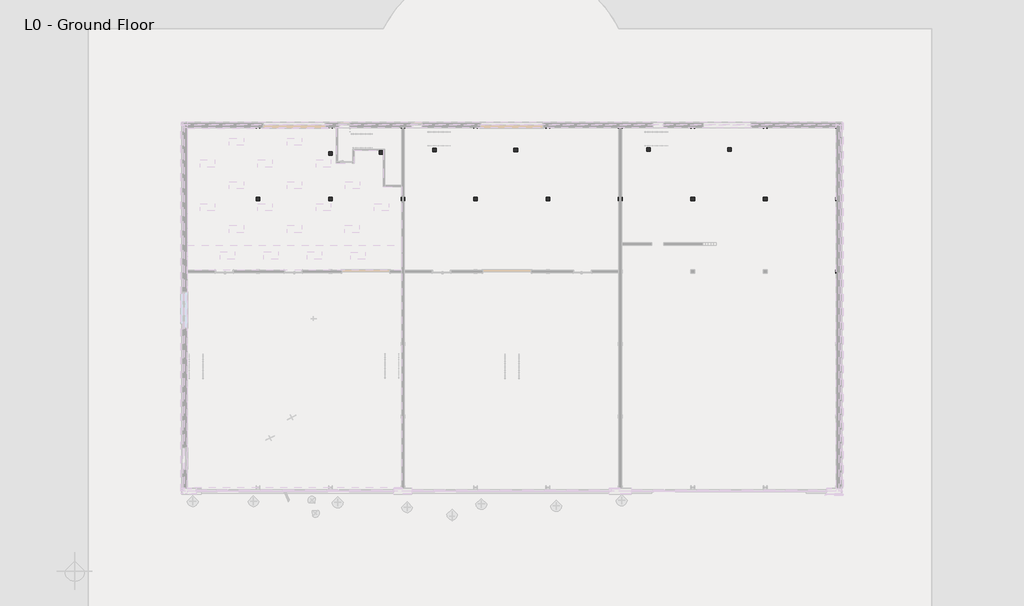
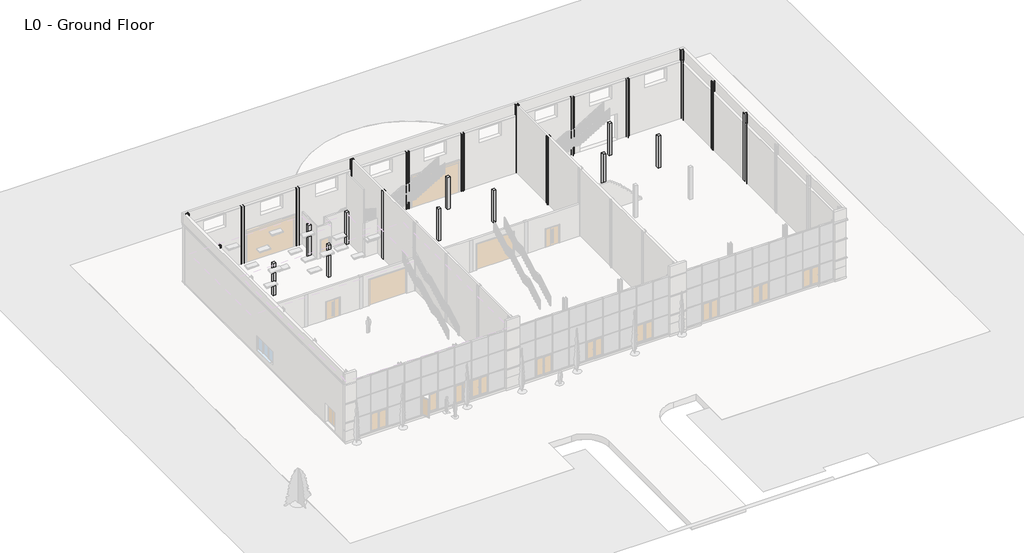
# One storey, part 7 of 14: 27 columns, 22 slabs, 2 footings.
"""IFC4 building model written with IfcOpenShell, lengths in millimetres."""

import ifcopenshell
import ifcopenshell.guid

model = None  # the IFC model being written
_history = None  # IfcOwnerHistory: only IFC2X3 demands one
_inside = {}  # id of a spatial element -> (the spatial element, [elements in it])
_under = {}  # id of a project, library or spatial element -> (it, [spatial elements below it])
_declared = {}  # id of a project -> (the project, [libraries it declares])
_typed = {}  # id of a type object -> (the type object, [elements of that type])
_made_of = {}  # id of a material, layer set ... -> (it, [elements and type objects made of it])


def new_model(schema):
    """Start an empty IFC model of exactly this schema.

    Asked for "IFC4X3", IfcOpenShell would pick the latest addendum, in which some entities
    have other attributes; the version numbers below select the first issue.
    IFC2X3 requires an IfcOwnerHistory on every rooted entity: one is made here for all.
    """
    global model, _history
    if schema == "IFC4X3":
        model = ifcopenshell.file(schema_version=(4, 3, 0, 0))
    else:
        model = ifcopenshell.file(schema=schema)
    _inside.clear()
    _under.clear()
    _declared.clear()
    _typed.clear()
    _made_of.clear()
    _history = None
    if model.schema == "IFC2X3":
        org = make("IfcOrganization", Name="unknown")
        user = make(
            "IfcPersonAndOrganization",
            ThePerson=make("IfcPerson", FamilyName="unknown"),
            TheOrganization=org,
        )
        app = make(
            "IfcApplication",
            ApplicationDeveloper=org,
            Version="unknown",
            ApplicationFullName="unknown",
            ApplicationIdentifier="unknown",
        )
        _history = make(
            "IfcOwnerHistory",
            OwningUser=user,
            OwningApplication=app,
            ChangeAction="ADDED",
            CreationDate=0,
        )
    return model


def make(cls, **values):
    """One entity of the class cls with the attributes given. An attribute that is None is left unset."""
    return model.create_entity(
        cls, **{name: value for name, value in values.items() if value is not None}
    )


def rooted(cls, **values):
    """An entity with a GlobalId (a new one), such as an element, a storey or a relation."""
    return make(cls, GlobalId=ifcopenshell.guid.new(), OwnerHistory=_history, **values)


def si_unit(unit_type, name, prefix=None):
    """IfcSIUnit, for example si_unit("LENGTHUNIT", "METRE", prefix="MILLI")."""
    return make("IfcSIUnit", UnitType=unit_type, Prefix=prefix, Name=name)


def assignment(units):
    """IfcUnitAssignment: the units of a project."""
    return None if units is None else make("IfcUnitAssignment", Units=units)


def point(xyz):
    """IfcCartesianPoint."""
    return None if xyz is None else make("IfcCartesianPoint", Coordinates=xyz)


def direction(xyz):
    """IfcDirection."""
    return None if xyz is None else make("IfcDirection", DirectionRatios=xyz)


def frame(location, z_axis=None, x_axis=None):
    """IfcAxis2Placement3D, a coordinate frame: its origin and axes. An axis left out is left unset."""
    return make(
        "IfcAxis2Placement3D",
        Location=point(location),
        Axis=direction(z_axis),
        RefDirection=direction(x_axis),
    )


def frame_2d(location, x_axis=None):
    """IfcAxis2Placement2D, a coordinate frame in the plane: its origin and x axis."""
    return make(
        "IfcAxis2Placement2D", Location=point(location), RefDirection=direction(x_axis)
    )


def origin():
    """The frame at (0, 0, 0) with its axes left unset."""
    return frame((0.0, 0.0, 0.0))


def place(relative_to, where):
    """IfcLocalPlacement: puts the frame where relative to a parent placement (None: the world)."""
    return make(
        "IfcLocalPlacement", PlacementRelTo=relative_to, RelativePlacement=where
    )


def context(
    kind, dimensions, precision=None, world=None, true_north=None, identifier=None
):
    """IfcGeometricRepresentationContext, for example the 3D "Model" context."""
    return make(
        "IfcGeometricRepresentationContext",
        ContextIdentifier=identifier,
        ContextType=kind,
        CoordinateSpaceDimension=dimensions,
        Precision=precision,
        WorldCoordinateSystem=world,
        TrueNorth=true_north,
    )


def project(units=None, contexts=None):
    """IfcProject with its units and contexts."""
    return rooted(
        "IfcProject",
        Name="project",
        RepresentationContexts=contexts,
        UnitsInContext=assignment(units),
    )


def spatial(cls, under=None, at=None, **own):
    """A site, building, storey or space (cls), placed at a placement, below another one or the project."""
    s = rooted(cls, ObjectPlacement=at, **own)
    if under is not None:
        _under.setdefault(under.id(), (under, []))[1].append(s)
    return s


def polyline(points):
    """IfcPolyline through the points."""
    return make("IfcPolyline", Points=[point(p) for p in points])


def circle_curve(where, radius):
    """IfcCircle in the frame where."""
    return make("IfcCircle", Position=where, Radius=radius)


def trimmed(basis, trim1, trim2, sense, master):
    """IfcTrimmedCurve: the piece of a basis curve between two trims."""
    return make(
        "IfcTrimmedCurve",
        BasisCurve=basis,
        Trim1=trim1,
        Trim2=trim2,
        SenseAgreement=sense,
        MasterRepresentation=master,
    )


def segment(curve, same_sense, transition):
    """IfcCompositeCurveSegment."""
    return make(
        "IfcCompositeCurveSegment",
        Transition=transition,
        SameSense=same_sense,
        ParentCurve=curve,
    )


def composite_curve(segments, self_intersect=None):
    """IfcCompositeCurve: segments joined end to end."""
    return make("IfcCompositeCurve", Segments=segments, SelfIntersect=self_intersect)


def outline(outer, holes=None, kind="AREA"):
    """IfcArbitraryClosedProfileDef: a profile drawn as a closed curve; with holes, ...WithVoids."""
    if holes is None:
        return make("IfcArbitraryClosedProfileDef", ProfileType=kind, OuterCurve=outer)
    return make(
        "IfcArbitraryProfileDefWithVoids",
        ProfileType=kind,
        OuterCurve=outer,
        InnerCurves=holes,
    )


def extrude(swept, where, along, depth):
    """IfcExtrudedAreaSolid: the profile swept, set in the frame where, extruded along a direction by depth."""
    return make(
        "IfcExtrudedAreaSolid",
        SweptArea=swept,
        Position=where,
        ExtrudedDirection=direction(along),
        Depth=depth,
    )


def faces_of(points, faces, orient=None, outer=None):
    """IfcFace entities. A face is a list of loops; a loop is a list of indices into points, from 0.

    orient and outer hold one flag for each loop. By default every Orientation is true, the
    first loop of a face is its IfcFaceOuterBound and the others are IfcFaceBound.
    """
    made = []
    for i, loops in enumerate(faces):
        bounds = []
        for j, loop in enumerate(loops):
            is_outer = j == 0 if outer is None else outer[i][j]
            bounds.append(
                make(
                    "IfcFaceOuterBound" if is_outer else "IfcFaceBound",
                    Bound=make("IfcPolyLoop", Polygon=[points[k] for k in loop]),
                    Orientation=True if orient is None else orient[i][j],
                )
            )
        made.append(make("IfcFace", Bounds=bounds))
    return made


def faceted_brep(points, faces, orient=None, outer=None, voids=None):
    """IfcFacetedBrep: a solid bounded by flat faces; with voids (closed shells), ...WithVoids."""
    shared = [point(p) for p in points]
    hull = make("IfcClosedShell", CfsFaces=faces_of(shared, faces, orient, outer))
    if voids is None:
        return make("IfcFacetedBrep", Outer=hull)
    return make(
        "IfcFacetedBrepWithVoids",
        Outer=hull,
        Voids=[
            make(cls, CfsFaces=faces_of(shared, fs, o, b)) for cls, fs, o, b in voids
        ],
    )


def shape(context_of_items, identifier, shape_type, items):
    """IfcShapeRepresentation: the items that make up one representation, for example the "Body"."""
    return make(
        "IfcShapeRepresentation",
        ContextOfItems=context_of_items,
        RepresentationIdentifier=identifier,
        RepresentationType=shape_type,
        Items=items,
    )


def source(mapping_origin, context_of_items, identifier, shape_type, items):
    """IfcRepresentationMap: a shape defined once, which mapped items show again and again."""
    return make(
        "IfcRepresentationMap",
        MappingOrigin=mapping_origin,
        MappedRepresentation=shape(context_of_items, identifier, shape_type, items),
    )


def transform(
    local_origin,
    x_axis=None,
    y_axis=None,
    z_axis=None,
    scale=None,
    scale2=None,
    scale3=None,
    uniform=True,
):
    """IfcCartesianTransformationOperator3D, or its non-uniform kind. x_axis, y_axis, z_axis: its Axis1, 2, 3."""
    if uniform:
        return make(
            "IfcCartesianTransformationOperator3D",
            Axis1=direction(x_axis),
            Axis2=direction(y_axis),
            LocalOrigin=point(local_origin),
            Scale=scale,
            Axis3=direction(z_axis),
        )
    return make(
        "IfcCartesianTransformationOperator3DnonUniform",
        Axis1=direction(x_axis),
        Axis2=direction(y_axis),
        LocalOrigin=point(local_origin),
        Scale=scale,
        Axis3=direction(z_axis),
        Scale2=scale2,
        Scale3=scale3,
    )


def mapped(mapping_source, mapping_target):
    """IfcMappedItem: shows the shape of a source again, moved by a transform."""
    return make(
        "IfcMappedItem", MappingSource=mapping_source, MappingTarget=mapping_target
    )


def made_of(thing, what):
    """Note that an element or type object is made of a material, layer set ...; save() writes the relation."""
    if what is not None:
        _made_of.setdefault(what.id(), (what, []))[1].append(thing)
    return thing


def element(
    cls,
    number,
    at=None,
    inside=None,
    cuts=None,
    type_object=None,
    material=None,
    context=None,
    identifier="Body",
    shape_type=None,
    held_by="IfcProductDefinitionShape",
    body=None,
    shapes=None,
    **own,
):
    """One element of the class cls, such as IfcWall. Its Tag is "e" and its number.

    at: its placement. inside: the storey or other place that contains it. cuts: it is an
    opening in that element (IfcRelVoidsElement). A single representation is given by context,
    identifier, shape_type and body (its items); several are given by shapes. held_by: the class
    of the entity that holds the representations. save() writes the other relations.
    """
    e = rooted(cls, Tag="e%d" % number, ObjectPlacement=at, **own)
    if body is not None:
        shapes = [shape(context, identifier, shape_type, body)]
    if shapes is not None:
        e.Representation = make(held_by, Representations=shapes)
    if inside is not None:
        _inside.setdefault(inside.id(), (inside, []))[1].append(e)
    if cuts is not None:
        rooted(
            "IfcRelVoidsElement", RelatingBuildingElement=cuts, RelatedOpeningElement=e
        )
    if type_object is not None:
        _typed.setdefault(type_object.id(), (type_object, []))[1].append(e)
    return made_of(e, material)


def aggregate(whole, parts):
    """IfcRelAggregates: a whole, such as a stair, and the parts it consists of."""
    return rooted("IfcRelAggregates", RelatingObject=whole, RelatedObjects=parts)


def save(model, path):
    """Write the relations noted so far, then the file.

    IfcRelAggregates (storeys below a building ...), IfcRelContainedInSpatialStructure (elements
    in a storey), IfcRelDefinesByType, IfcRelAssociatesMaterial and IfcRelDeclares: one each for
    every whole, place, type object, material and project.
    """
    for whole, parts in _under.values():
        aggregate(whole, parts)
    for where, things in _inside.values():
        rooted(
            "IfcRelContainedInSpatialStructure",
            RelatedElements=things,
            RelatingStructure=where,
        )
    for kind, things in _typed.values():
        rooted("IfcRelDefinesByType", RelatedObjects=things, RelatingType=kind)
    for what, things in _made_of.values():
        rooted("IfcRelAssociatesMaterial", RelatedObjects=things, RelatingMaterial=what)
    for by, libraries in _declared.values():
        rooted("IfcRelDeclares", RelatingContext=by, RelatedDefinitions=libraries)
    model.write(path)


def uc_universal_column_column_305x305x97uc_f4bfb62a(model_context):
    return source(origin(), model_context, "Body", "SweptSolid", [
        extrude(outline(composite_curve([segment(polyline([(152.65, 153.95), (152.65, 138.55), (20.15, 138.55)]), True, "CONTINUOUS"), segment(trimmed(circle_curve(frame_2d((20.15, 123.35)), 15.2), [point((20.15, 138.55))], [point((4.95, 123.35))], True, "CARTESIAN"), True, "CONTINUOUS"), segment(polyline([(4.95, 123.35), (4.95, -123.35)]), True, "CONTINUOUS"), segment(trimmed(circle_curve(frame_2d((20.15, -123.35)), 15.2), [point((4.95, -123.35))], [point((20.15, -138.55))], True, "CARTESIAN"), True, "CONTINUOUS"), segment(polyline([(20.15, -138.55), (152.65, -138.55), (152.65, -153.95), (-152.65, -153.95), (-152.65, -138.55), (-20.15, -138.55)]), True, "CONTINUOUS"), segment(trimmed(circle_curve(frame_2d((-20.15, -123.35)), 15.2), [point((-20.15, -138.55))], [point((-4.95, -123.35))], True, "CARTESIAN"), True, "CONTINUOUS"), segment(polyline([(-4.95, -123.35), (-4.95, 123.35)]), True, "CONTINUOUS"), segment(trimmed(circle_curve(frame_2d((-20.15, 123.35)), 15.2), [point((-4.95, 123.35))], [point((-20.15, 138.55))], True, "CARTESIAN"), True, "CONTINUOUS"), segment(polyline([(-20.15, 138.55), (-152.65, 138.55), (-152.65, 153.95), (152.65, 153.95)]), True, "CONTINUOUS")], self_intersect=False)), frame((0.0, 0.0, -1500.0), z_axis=(0.0, 0.0, 1.0), x_axis=(1.0, 0.0, 0.0)), (0.0, 0.0, 1.0), 9300.0),
    ])


def uc_universal_column_column_305x305x97uc_8da79b43(model_context):
    return source(origin(), model_context, "Body", "SweptSolid", [
        extrude(outline(composite_curve([segment(polyline([(152.65, -153.95), (-152.65, -153.95), (-152.65, -138.55), (-20.15, -138.55)]), True, "CONTINUOUS"), segment(trimmed(circle_curve(frame_2d((-20.15, -123.35)), 15.2), [point((-20.15, -138.55))], [point((-4.95, -123.35))], True, "CARTESIAN"), True, "CONTINUOUS"), segment(polyline([(-4.95, -123.35), (-4.95, 123.35)]), True, "CONTINUOUS"), segment(trimmed(circle_curve(frame_2d((-20.15, 123.35)), 15.2), [point((-4.95, 123.35))], [point((-20.15, 138.55))], True, "CARTESIAN"), True, "CONTINUOUS"), segment(polyline([(-20.15, 138.55), (-152.65, 138.55), (-152.65, 153.95), (152.65, 153.95), (152.65, 138.55), (20.15, 138.55)]), True, "CONTINUOUS"), segment(trimmed(circle_curve(frame_2d((20.15, 123.35)), 15.2), [point((20.15, 138.55))], [point((4.95, 123.35))], True, "CARTESIAN"), True, "CONTINUOUS"), segment(polyline([(4.95, 123.35), (4.95, -123.35)]), True, "CONTINUOUS"), segment(trimmed(circle_curve(frame_2d((20.15, -123.35)), 15.2), [point((4.95, -123.35))], [point((20.15, -138.55))], True, "CARTESIAN"), True, "CONTINUOUS"), segment(polyline([(20.15, -138.55), (152.65, -138.55), (152.65, -153.95)]), True, "CONTINUOUS")], self_intersect=False)), frame((0.0, 0.0, -1500.0), z_axis=(0.0, 0.0, 1.0), x_axis=(1.0, 0.0, 0.0)), (0.0, 0.0, 1.0), 9300.0),
    ])


def uc_universal_column_column_305x305x97uc_43a052ce(model_context):
    return source(origin(), model_context, "Body", "SweptSolid", [
        extrude(outline(composite_curve([segment(polyline([(152.65, 153.95), (152.65, 138.55), (20.15, 138.55)]), True, "CONTINUOUS"), segment(trimmed(circle_curve(frame_2d((20.15, 123.35)), 15.2), [point((20.15, 138.55))], [point((4.95, 123.35))], True, "CARTESIAN"), True, "CONTINUOUS"), segment(polyline([(4.95, 123.35), (4.95, -123.35)]), True, "CONTINUOUS"), segment(trimmed(circle_curve(frame_2d((20.15, -123.35)), 15.2), [point((4.95, -123.35))], [point((20.15, -138.55))], True, "CARTESIAN"), True, "CONTINUOUS"), segment(polyline([(20.15, -138.55), (152.65, -138.55), (152.65, -153.95), (-152.65, -153.95), (-152.65, -138.55), (-20.15, -138.55)]), True, "CONTINUOUS"), segment(trimmed(circle_curve(frame_2d((-20.15, -123.35)), 15.2), [point((-20.15, -138.55))], [point((-4.95, -123.35))], True, "CARTESIAN"), True, "CONTINUOUS"), segment(polyline([(-4.95, -123.35), (-4.95, 123.35)]), True, "CONTINUOUS"), segment(trimmed(circle_curve(frame_2d((-20.15, 123.35)), 15.2), [point((-4.95, 123.35))], [point((-20.15, 138.55))], True, "CARTESIAN"), True, "CONTINUOUS"), segment(polyline([(-20.15, 138.55), (-152.65, 138.55), (-152.65, 153.95), (152.65, 153.95)]), True, "CONTINUOUS")], self_intersect=False)), frame((0.0, 0.0, -1500.0), z_axis=(0.0, 0.0, 1.0), x_axis=(1.0, 0.0, 0.0)), (0.0, 0.0, 1.0), 8100.0),
    ])


def pad_foundation_rectangular_1000x1000x500_ed6229e9(model_context):
    return source(origin(), model_context, "Body", "SweptSolid", [
        extrude(outline(polyline([(500.0, 500.0), (500.0, -500.0), (-500.0, -500.0), (-500.0, 500.0), (500.0, 500.0)])), frame((0.0, 0.0, -500.0), z_axis=(0.0, 0.0, 1.0), x_axis=(1.0, 0.0, 0.0)), (0.0, 0.0, 1.0), 500.0),
    ])


model = new_model("IFC4")

# Units and contexts
model_context = context("Model", 3, world=origin())
ifc_project = project(units=[si_unit("LENGTHUNIT", "METRE", prefix="MILLI")], contexts=[model_context])

# Site, building, storey
site = spatial("IfcSite", under=ifc_project)
building = spatial("IfcBuilding", under=site)
storey = spatial("IfcBuildingStorey", under=building, Name="L0 - Ground Floor", Elevation=0.0)

# Columns
placement = place(None, origin())
element("IfcColumn", 1, ObjectType="Concrete Square : 300 x 300mm", at=placement, inside=storey, context=model_context, shape_type="SweptSolid", body=[
    extrude(outline(polyline([(-989.5553457, 791.2380918), (-1289.5553457, 791.2380918), (-1289.5553457, 1091.2380918), (-989.5553457, 1091.2380918), (-989.5553457, 791.2380918)])), frame((0.0, 0.0, -1500.0), z_axis=(0.0, 0.0, 1.0), x_axis=(1.0, 0.0, 0.0)), (0.0, 0.0, 1.0), 5200.0),
])
element("IfcColumn", 2, ObjectType="Concrete Square : 300 x 300mm", at=placement, inside=storey, context=model_context, shape_type="SweptSolid", body=[
    extrude(outline(polyline([(9194.5066977, 4635.3001351), (8894.5066977, 4635.3001351), (8894.5066977, 4935.3001351), (9194.5066977, 4935.3001351), (9194.5066977, 4635.3001351)])), frame((0.0, 0.0, -1500.0), z_axis=(0.0, 0.0, 1.0), x_axis=(1.0, 0.0, 0.0)), (0.0, 0.0, 1.0), 5200.0),
])
element("IfcColumn", 3, ObjectType="Concrete Square : 300 x 300mm", at=placement, inside=storey, context=model_context, shape_type="SweptSolid", body=[
    extrude(outline(polyline([(17010.4446543, 791.2380918), (16710.4446543, 791.2380918), (16710.4446543, 1091.2380918), (17010.4446543, 1091.2380918), (17010.4446543, 791.2380918)])), frame((0.0, 0.0, -1500.0), z_axis=(0.0, 0.0, 1.0), x_axis=(1.0, 0.0, 0.0)), (0.0, 0.0, 1.0), 5200.0),
])
element("IfcColumn", 4, ObjectType="Concrete Square : 300 x 300mm", at=placement, inside=storey, context=model_context, shape_type="SweptSolid", body=[
    extrude(outline(polyline([(23010.4446543, 791.2380918), (22710.4446543, 791.2380918), (22710.4446543, 1091.2380918), (23010.4446543, 1091.2380918), (23010.4446543, 791.2380918)])), frame((0.0, 0.0, -1500.0), z_axis=(0.0, 0.0, 1.0), x_axis=(1.0, 0.0, 0.0)), (0.0, 0.0, 1.0), 5200.0),
])
element("IfcColumn", 5, ObjectType="Concrete Square : 300 x 300mm", at=placement, inside=storey, context=model_context, shape_type="SweptSolid", body=[
    extrude(outline(polyline([(35010.4446543, 791.2380918), (34710.4446543, 791.2380918), (34710.4446543, 1091.2380918), (35010.4446543, 1091.2380918), (35010.4446543, 791.2380918)])), frame((0.0, 0.0, -1500.0), z_axis=(0.0, 0.0, 1.0), x_axis=(1.0, 0.0, 0.0)), (0.0, 0.0, 1.0), 5200.0),
])
element("IfcColumn", 6, ObjectType="Concrete Square : 300 x 300mm", at=placement, inside=storey, context=model_context, shape_type="SweptSolid", body=[
    extrude(outline(polyline([(41010.4446543, 791.2380918), (40710.4446543, 791.2380918), (40710.4446543, 1091.2380918), (41010.4446543, 1091.2380918), (41010.4446543, 791.2380918)])), frame((0.0, 0.0, -1500.0), z_axis=(0.0, 0.0, 1.0), x_axis=(1.0, 0.0, 0.0)), (0.0, 0.0, 1.0), 5200.0),
])
element("IfcColumn", 7, ObjectType="Concrete Square : 300 x 300mm", at=placement, inside=storey, context=model_context, shape_type="SweptSolid", body=[
    extrude(outline(polyline([(5010.4446543, 791.2380918), (4710.4446543, 791.2380918), (4710.4446543, 1091.2380918), (5010.4446543, 1091.2380918), (5010.4446543, 791.2380918)])), frame((0.0, 0.0, -1500.0), z_axis=(0.0, 0.0, 1.0), x_axis=(1.0, 0.0, 0.0)), (0.0, 0.0, 1.0), 5200.0),
])
element("IfcColumn", 8, ObjectType="Concrete Square : 300 x 300mm", at=placement, inside=storey, context=model_context, shape_type="SweptSolid", body=[
    extrude(outline(polyline([(5022.9446543, 4575.3001351), (4722.9446543, 4575.3001351), (4722.9446543, 4875.3001351), (5022.9446543, 4875.3001351), (5022.9446543, 4575.3001351)])), frame((0.0, 0.0, -1500.0), z_axis=(0.0, 0.0, 1.0), x_axis=(1.0, 0.0, 0.0)), (0.0, 0.0, 1.0), 5200.0),
])
element("IfcColumn", 9, ObjectType="Concrete Square : 300 x 300mm", at=placement, inside=storey, context=model_context, shape_type="SweptSolid", body=[
    extrude(outline(polyline([(20350.4446543, 4850.3001351), (20050.4446543, 4850.3001351), (20050.4446543, 5150.3001351), (20350.4446543, 5150.3001351), (20350.4446543, 4850.3001351)])), frame((0.0, 0.0, -1500.0), z_axis=(0.0, 0.0, 1.0), x_axis=(1.0, 0.0, 0.0)), (0.0, 0.0, 1.0), 5200.0),
])
element("IfcColumn", 10, ObjectType="Concrete Square : 300 x 300mm", at=placement, inside=storey, context=model_context, shape_type="SweptSolid", body=[
    extrude(outline(polyline([(13627.9446543, 5150.3001351), (13627.9446543, 4850.3001351), (13327.9446543, 4850.3001351), (13327.9446543, 5150.3001351), (13627.9446543, 5150.3001351)])), frame((0.0, 0.0, -1500.0), z_axis=(0.0, 0.0, 1.0), x_axis=(1.0, 0.0, 0.0)), (0.0, 0.0, 1.0), 5200.0),
])
element("IfcColumn", 11, ObjectType="Concrete Square : 300 x 300mm", at=placement, inside=storey, context=model_context, shape_type="SweptSolid", body=[
    extrude(outline(polyline([(31350.4446543, 4891.2380918), (31050.4446543, 4891.2380918), (31050.4446543, 5191.2380918), (31350.4446543, 5191.2380918), (31350.4446543, 4891.2380918)])), frame((0.0, 0.0, -1500.0), z_axis=(0.0, 0.0, 1.0), x_axis=(1.0, 0.0, 0.0)), (0.0, 0.0, 1.0), 5200.0),
])
element("IfcColumn", 12, ObjectType="Concrete Square : 300 x 300mm", at=placement, inside=storey, context=model_context, shape_type="SweptSolid", body=[
    extrude(outline(polyline([(38050.4446543, 4891.2380918), (37750.4446543, 4891.2380918), (37750.4446543, 5191.2380918), (38050.4446543, 5191.2380918), (38050.4446543, 4891.2380918)])), frame((0.0, 0.0, -1500.0), z_axis=(0.0, 0.0, 1.0), x_axis=(1.0, 0.0, 0.0)), (0.0, 0.0, 1.0), 5200.0),
])
element("IfcColumn", 13, ObjectType="UC-Universal Column-Column : 305x305x97UC", at=placement, inside=storey, context=model_context, shape_type="SweptSolid", body=[
    extrude(outline(composite_curve([segment(polyline([(-7293.5053457, 1093.8880918), (-7278.1053457, 1093.8880918), (-7278.1053457, 961.3880918)]), True, "CONTINUOUS"), segment(trimmed(circle_curve(frame_2d((-7262.9053457, 961.3880918)), 15.2), [point((-7278.1053457, 961.3880918))], [point((-7262.9053457, 946.1880918))], True, "CARTESIAN"), True, "CONTINUOUS"), segment(polyline([(-7262.9053457, 946.1880918), (-7016.2053457, 946.1880918)]), True, "CONTINUOUS"), segment(trimmed(circle_curve(frame_2d((-7016.2053457, 961.3880918)), 15.2), [point((-7016.2053457, 946.1880918))], [point((-7001.0053457, 961.3880918))], True, "CARTESIAN"), True, "CONTINUOUS"), segment(polyline([(-7001.0053457, 961.3880918), (-7001.0053457, 1093.8880918), (-6985.6053457, 1093.8880918), (-6985.6053457, 788.5880918), (-7001.0053457, 788.5880918), (-7001.0053457, 921.0880918)]), True, "CONTINUOUS"), segment(trimmed(circle_curve(frame_2d((-7016.2053457, 921.0880918)), 15.2), [point((-7001.0053457, 921.0880918))], [point((-7016.2053457, 936.2880918))], True, "CARTESIAN"), True, "CONTINUOUS"), segment(polyline([(-7016.2053457, 936.2880918), (-7262.9053457, 936.2880918)]), True, "CONTINUOUS"), segment(trimmed(circle_curve(frame_2d((-7262.9053457, 921.0880918)), 15.2), [point((-7262.9053457, 936.2880918))], [point((-7278.1053457, 921.0880918))], True, "CARTESIAN"), True, "CONTINUOUS"), segment(polyline([(-7278.1053457, 921.0880918), (-7278.1053457, 788.5880918), (-7293.5053457, 788.5880918), (-7293.5053457, 1093.8880918)]), True, "CONTINUOUS")], self_intersect=False)), frame((0.0, 0.0, -1500.0), z_axis=(0.0, 0.0, 1.0), x_axis=(1.0, 0.0, 0.0)), (0.0, 0.0, 1.0), 9300.0),
])
uc_universal_column_column_305x305x97uc_shape = uc_universal_column_column_305x305x97uc_f4bfb62a(model_context)
element("IfcColumn", 14, ObjectType="UC-Universal Column-Column : 305x305x97UC", at=placement, inside=storey, context=model_context, shape_type="MappedRepresentation", body=[
    mapped(uc_universal_column_column_305x305x97uc_shape, transform((-7139.5553457, 6941.2380918, 0.0), x_axis=(0.0, 1.0, 0.0), y_axis=(-1.0, 0.0, 0.0), z_axis=(0.0, 0.0, 1.0))),
])
element("IfcColumn", 15, ObjectType="UC-Universal Column-Column : 305x305x97UC", at=placement, inside=storey, context=model_context, shape_type="MappedRepresentation", body=[
    mapped(uc_universal_column_column_305x305x97uc_shape, transform((10860.4446543, 6941.2380918, 0.0), x_axis=(0.0, 1.0, 0.0), y_axis=(-1.0, 0.0, 0.0), z_axis=(0.0, 0.0, 1.0))),
])
element("IfcColumn", 16, ObjectType="UC-Universal Column-Column : 305x305x97UC", at=placement, inside=storey, context=model_context, shape_type="MappedRepresentation", body=[
    mapped(uc_universal_column_column_305x305x97uc_shape, transform((28860.4446543, 6941.2380918, 0.0), x_axis=(0.0, 1.0, 0.0), y_axis=(-1.0, 0.0, 0.0), z_axis=(0.0, 0.0, 1.0))),
])
element("IfcColumn", 17, ObjectType="UC-Universal Column-Column : 305x305x97UC", at=placement, inside=storey, context=model_context, shape_type="MappedRepresentation", body=[
    mapped(uc_universal_column_column_305x305x97uc_shape, transform((10860.4446543, 941.2380918, 0.0), x_axis=(0.0, 1.0, 0.0), y_axis=(-1.0, 0.0, 0.0), z_axis=(0.0, 0.0, 1.0))),
])
element("IfcColumn", 18, ObjectType="UC-Universal Column-Column : 305x305x97UC", at=placement, inside=storey, context=model_context, shape_type="MappedRepresentation", body=[
    mapped(uc_universal_column_column_305x305x97uc_shape, transform((28860.4446543, 941.2380918, 0.0), x_axis=(0.0, 1.0, 0.0), y_axis=(-1.0, 0.0, 0.0), z_axis=(0.0, 0.0, 1.0))),
])
uc_universal_column_column_305x305x97uc_2_shape = uc_universal_column_column_305x305x97uc_8da79b43(model_context)
element("IfcColumn", 19, ObjectType="UC-Universal Column-Column : 305x305x97UC", at=placement, inside=storey, context=model_context, shape_type="MappedRepresentation", body=[
    mapped(uc_universal_column_column_305x305x97uc_2_shape, transform((46860.4446543, -5058.7619082, 0.0), x_axis=(0.0, 1.0, 0.0), y_axis=(-1.0, 0.0, 0.0), z_axis=(0.0, 0.0, 1.0))),
])
element("IfcColumn", 20, ObjectType="UC-Universal Column-Column : 305x305x97UC", at=placement, inside=storey, context=model_context, shape_type="MappedRepresentation", body=[
    mapped(uc_universal_column_column_305x305x97uc_2_shape, transform((46860.4446543, 941.2380918, 0.0), x_axis=(0.0, 1.0, 0.0), y_axis=(-1.0, 0.0, 0.0), z_axis=(0.0, 0.0, 1.0))),
])
element("IfcColumn", 21, ObjectType="UC-Universal Column-Column : 305x305x97UC", at=placement, inside=storey, context=model_context, shape_type="MappedRepresentation", body=[
    mapped(uc_universal_column_column_305x305x97uc_2_shape, transform((46860.4446543, 6941.2380918, 0.0), x_axis=(0.0, 1.0, 0.0), y_axis=(-1.0, 0.0, 0.0), z_axis=(0.0, 0.0, 1.0))),
])
uc_universal_column_column_305x305x97uc_3_shape = uc_universal_column_column_305x305x97uc_43a052ce(model_context)
element("IfcColumn", 22, ObjectType="UC-Universal Column-Column : 305x305x97UC", at=placement, inside=storey, context=model_context, shape_type="MappedRepresentation", body=[
    mapped(uc_universal_column_column_305x305x97uc_3_shape, transform((-1139.5553457, 6941.2380918, 0.0), x_axis=(0.0, 1.0, 0.0), y_axis=(-1.0, 0.0, 0.0), z_axis=(0.0, 0.0, 1.0))),
])
element("IfcColumn", 23, ObjectType="UC-Universal Column-Column : 305x305x97UC", at=placement, inside=storey, context=model_context, shape_type="MappedRepresentation", body=[
    mapped(uc_universal_column_column_305x305x97uc_3_shape, transform((4860.4446543, 6941.2380918, 0.0), x_axis=(0.0, 1.0, 0.0), y_axis=(-1.0, 0.0, 0.0), z_axis=(0.0, 0.0, 1.0))),
])
element("IfcColumn", 24, ObjectType="UC-Universal Column-Column : 305x305x97UC", at=placement, inside=storey, context=model_context, shape_type="MappedRepresentation", body=[
    mapped(uc_universal_column_column_305x305x97uc_3_shape, transform((16860.4446543, 6941.2380918, 0.0), x_axis=(0.0, 1.0, 0.0), y_axis=(-1.0, 0.0, 0.0), z_axis=(0.0, 0.0, 1.0))),
])
element("IfcColumn", 25, ObjectType="UC-Universal Column-Column : 305x305x97UC", at=placement, inside=storey, context=model_context, shape_type="MappedRepresentation", body=[
    mapped(uc_universal_column_column_305x305x97uc_3_shape, transform((22860.4446543, 6941.2380918, 0.0), x_axis=(0.0, 1.0, 0.0), y_axis=(-1.0, 0.0, 0.0), z_axis=(0.0, 0.0, 1.0))),
])
element("IfcColumn", 26, ObjectType="UC-Universal Column-Column : 305x305x97UC", at=placement, inside=storey, context=model_context, shape_type="MappedRepresentation", body=[
    mapped(uc_universal_column_column_305x305x97uc_3_shape, transform((34860.4446543, 6941.2380918, 0.0), x_axis=(0.0, 1.0, 0.0), y_axis=(-1.0, 0.0, 0.0), z_axis=(0.0, 0.0, 1.0))),
])
element("IfcColumn", 27, ObjectType="UC-Universal Column-Column : 305x305x97UC", at=placement, inside=storey, context=model_context, shape_type="MappedRepresentation", body=[
    mapped(uc_universal_column_column_305x305x97uc_3_shape, transform((40860.4446543, 6941.2380918, 0.0), x_axis=(0.0, 1.0, 0.0), y_axis=(-1.0, 0.0, 0.0), z_axis=(0.0, 0.0, 1.0))),
])

# Footings
element("IfcFooting", 28, ObjectType="Wall Foundation - Commercial 1300 x 450", at=placement, inside=storey, context=model_context, shape_type="Brep", body=[
    faceted_brep([(47425.1446543, 7505.9380918, -1200.0), (46510.7446543, 7505.9380918, -1200.0), (46510.7446543, 6591.5380918, -1200.0), (46510.7446543, -22819.0474846, -1200.0), (47425.1446543, -22819.0474846, -1200.0), (47425.1446543, 7505.9380918, -1504.8), (47425.1446543, -22819.0474846, -1504.8), (46510.7446543, 7505.9380918, -1504.8), (47360.4446543, -22819.0474846, -1504.8), (47360.4446543, -22448.7619082, -1504.8), (46510.7446543, -22448.7619082, -1504.8), (46510.7446543, -17558.7619082, -1504.8), (47360.4446543, -17558.7619082, -1504.8), (47360.4446543, -16558.7619082, -1504.8), (46510.7446543, -16558.7619082, -1504.8), (46510.7446543, -11558.7619082, -1504.8), (47360.4446543, -11558.7619082, -1504.8), (47360.4446543, -10558.7619082, -1504.8), (46510.7446543, -10558.7619082, -1504.8), (46510.7446543, -5558.7619082, -1504.8), (47360.4446543, -5558.7619082, -1504.8), (47360.4446543, -4558.7619082, -1504.8), (46510.7446543, -4558.7619082, -1504.8), (46510.7446543, 441.2380918, -1504.8), (47360.4446543, 441.2380918, -1504.8), (47360.4446543, 1441.2380918, -1504.8), (46510.7446543, 1441.2380918, -1504.8), (46510.7446543, 6441.2380918, -1504.8), (47360.4446543, 6441.2380918, -1504.8), (47360.4446543, 7441.2380918, -1504.8), (46510.7446543, 7441.2380918, -1504.8), (46510.7446543, 7441.2380918, -1500.0), (46510.7446543, 6591.5380918, -1500.0), (46510.7446543, 6441.2380918, -1500.0), (46510.7446543, 1441.2380918, -1500.0), (46510.7446543, 441.2380918, -1500.0), (46510.7446543, -4558.7619082, -1500.0), (46510.7446543, -5558.7619082, -1500.0), (46510.7446543, -10558.7619082, -1500.0), (46510.7446543, -11558.7619082, -1500.0), (46510.7446543, -16558.7619082, -1500.0), (46510.7446543, -17558.7619082, -1500.0), (46510.7446543, -22448.7619082, -1500.0), (46510.7446543, -22819.0474846, -1500.0), (47360.4446543, 1441.2380918, -1500.0), (47360.4446543, 441.2380918, -1500.0), (47360.4446543, 7441.2380918, -1500.0), (47360.4446543, 6441.2380918, -1500.0), (47360.4446543, -4558.7619082, -1500.0), (47360.4446543, -5558.7619082, -1500.0), (47360.4446543, -10558.7619082, -1500.0), (47360.4446543, -11558.7619082, -1500.0), (47360.4446543, -16558.7619082, -1500.0), (47360.4446543, -17558.7619082, -1500.0), (47360.4446543, -22448.7619082, -1500.0), (47360.4446543, -22819.0474846, -1500.0)], [[[0, 1, 2, 3, 4]], [[5, 0, 4, 6]], [[7, 5, 6, 8, 9, 10, 11, 12, 13, 14, 15, 16, 17, 18, 19, 20, 21, 22, 23, 24, 25, 26, 27, 28, 29, 30]], [[1, 7, 30, 31, 32, 33, 27, 26, 34, 35, 23, 22, 36, 37, 19, 18, 38, 39, 15, 14, 40, 41, 11, 10, 42, 43, 3, 2]], [[1, 0, 5, 7]], [[44, 45, 35, 34]], [[44, 34, 26, 25]], [[35, 45, 24, 23]], [[45, 44, 25, 24]], [[46, 47, 33, 32, 31]], [[33, 47, 28, 27]], [[47, 46, 29, 28]], [[48, 49, 37, 36]], [[48, 36, 22, 21]], [[37, 49, 20, 19]], [[49, 48, 21, 20]], [[50, 51, 39, 38]], [[50, 38, 18, 17]], [[39, 51, 16, 15]], [[51, 50, 17, 16]], [[52, 53, 41, 40]], [[52, 40, 14, 13]], [[41, 53, 12, 11]], [[53, 52, 13, 12]], [[42, 54, 55, 43]], [[54, 42, 10, 9]], [[54, 9, 8, 55]], [[4, 3, 43, 55, 8, 6]], [[46, 31, 30, 29]]]),
])
element("IfcFooting", 29, ObjectType="Wall Foundation - Commercial 1300 x 450", at=placement, inside=storey, context=model_context, shape_type="Brep", body=[
    faceted_brep([(46510.7446543, 6591.5380918, -1200.0), (46510.7446543, 7505.9380918, -1200.0), (-6758.8053457, 7505.9380918, -1200.0), (-6758.8053457, 6591.5380918, -1200.0), (10403.2446543, 6591.5380918, -1200.0), (11317.6446543, 6591.5380918, -1200.0), (28403.2446543, 6591.5380918, -1200.0), (29317.6446543, 6591.5380918, -1200.0), (46510.7446543, 7505.9380918, -1504.8), (-6758.8053457, 7505.9380918, -1504.8), (41386.4946543, 7441.2380918, -1504.8), (40386.4946543, 7441.2380918, -1504.8), (40386.4946543, 6591.5380918, -1504.8), (35347.9446543, 6591.5380918, -1504.8), (35347.9446543, 7441.2380918, -1504.8), (34347.9446543, 7441.2380918, -1504.8), (34347.9446543, 6591.5380918, -1504.8), (29360.4446543, 6591.5380918, -1504.8), (29360.4446543, 7441.2380918, -1504.8), (28360.4446543, 7441.2380918, -1504.8), (28360.4446543, 6591.5380918, -1504.8), (23360.4446543, 6591.5380918, -1504.8), (23360.4446543, 7441.2380918, -1504.8), (22360.4446543, 7441.2380918, -1504.8), (22360.4446543, 6591.5380918, -1504.8), (17360.4446543, 6591.5380918, -1504.8), (17360.4446543, 7441.2380918, -1504.8), (16360.4446543, 7441.2380918, -1504.8), (16360.4446543, 6591.5380918, -1504.8), (11360.4446543, 6591.5380918, -1504.8), (11360.4446543, 7441.2380918, -1504.8), (10360.4446543, 7441.2380918, -1504.8), (10360.4446543, 6591.5380918, -1504.8), (5360.4446543, 6591.5380918, -1504.8), (5360.4446543, 7441.2380918, -1504.8), (4360.4446543, 7441.2380918, -1504.8), (4360.4446543, 6591.5380918, -1504.8), (-639.5553457, 6591.5380918, -1504.8), (-639.5553457, 7441.2380918, -1504.8), (-1639.5553457, 7441.2380918, -1504.8), (-1639.5553457, 6591.5380918, -1504.8), (-6639.5553457, 6591.5380918, -1504.8), (-6639.5553457, 7441.2380918, -1504.8), (-6758.8053457, 7441.2380918, -1504.8), (46510.7446543, 7441.2380918, -1504.8), (46360.4446543, 7441.2380918, -1504.8), (46360.4446543, 6591.5380918, -1504.8), (41386.4946543, 6591.5380918, -1504.8), (40386.4946543, 6591.5380918, -1500.0), (41386.4946543, 6591.5380918, -1500.0), (46360.4446543, 6591.5380918, -1500.0), (46510.7446543, 6591.5380918, -1500.0), (-6758.8053457, 6591.5380918, -1500.0), (-6639.5553457, 6591.5380918, -1500.0), (-1639.5553457, 6591.5380918, -1500.0), (-639.5553457, 6591.5380918, -1500.0), (4360.4446543, 6591.5380918, -1500.0), (5360.4446543, 6591.5380918, -1500.0), (10360.4446543, 6591.5380918, -1500.0), (10403.2446543, 6591.5380918, -1500.0), (11317.6446543, 6591.5380918, -1500.0), (11360.4446543, 6591.5380918, -1500.0), (16360.4446543, 6591.5380918, -1500.0), (17360.4446543, 6591.5380918, -1500.0), (22360.4446543, 6591.5380918, -1500.0), (23360.4446543, 6591.5380918, -1500.0), (28360.4446543, 6591.5380918, -1500.0), (28403.2446543, 6591.5380918, -1500.0), (29317.6446543, 6591.5380918, -1500.0), (29360.4446543, 6591.5380918, -1500.0), (34347.9446543, 6591.5380918, -1500.0), (35347.9446543, 6591.5380918, -1500.0), (40386.4946543, 7441.2380918, -1500.0), (41386.4946543, 7441.2380918, -1500.0), (34347.9446543, 7441.2380918, -1500.0), (35347.9446543, 7441.2380918, -1500.0), (28360.4446543, 7441.2380918, -1500.0), (29360.4446543, 7441.2380918, -1500.0), (22360.4446543, 7441.2380918, -1500.0), (23360.4446543, 7441.2380918, -1500.0), (16360.4446543, 7441.2380918, -1500.0), (17360.4446543, 7441.2380918, -1500.0), (10360.4446543, 7441.2380918, -1500.0), (11360.4446543, 7441.2380918, -1500.0), (4360.4446543, 7441.2380918, -1500.0), (5360.4446543, 7441.2380918, -1500.0), (-1639.5553457, 7441.2380918, -1500.0), (-639.5553457, 7441.2380918, -1500.0), (-6639.5553457, 7441.2380918, -1500.0), (-6758.8053457, 7441.2380918, -1500.0), (46510.7446543, 7441.2380918, -1500.0), (46360.4446543, 7441.2380918, -1500.0)], [[[0, 1, 2, 3, 4, 5, 6, 7]], [[1, 8, 9, 2]], [[10, 11, 12, 13, 14, 15, 16, 17, 18, 19, 20, 21, 22, 23, 24, 25, 26, 27, 28, 29, 30, 31, 32, 33, 34, 35, 36, 37, 38, 39, 40, 41, 42, 43, 9, 8, 44, 45, 46, 47]], [[48, 49, 47, 46, 50, 51, 0, 7, 6, 5, 4, 3, 52, 53, 41, 40, 54, 55, 37, 36, 56, 57, 33, 32, 58, 59, 60, 61, 29, 28, 62, 63, 25, 24, 64, 65, 21, 20, 66, 67, 68, 69, 17, 16, 70, 71, 13, 12]], [[72, 73, 49, 48]], [[73, 72, 11, 10]], [[72, 48, 12, 11]], [[49, 73, 10, 47]], [[74, 75, 71, 70]], [[75, 74, 15, 14]], [[74, 70, 16, 15]], [[71, 75, 14, 13]], [[76, 77, 69, 68, 67, 66]], [[77, 76, 19, 18]], [[76, 66, 20, 19]], [[69, 77, 18, 17]], [[78, 79, 65, 64]], [[79, 78, 23, 22]], [[78, 64, 24, 23]], [[65, 79, 22, 21]], [[80, 81, 63, 62]], [[81, 80, 27, 26]], [[80, 62, 28, 27]], [[63, 81, 26, 25]], [[82, 83, 61, 60, 59, 58]], [[83, 82, 31, 30]], [[82, 58, 32, 31]], [[61, 83, 30, 29]], [[84, 85, 57, 56]], [[85, 84, 35, 34]], [[84, 56, 36, 35]], [[57, 85, 34, 33]], [[86, 87, 55, 54]], [[87, 86, 39, 38]], [[86, 54, 40, 39]], [[55, 87, 38, 37]], [[88, 53, 52, 89]], [[42, 88, 89, 43]], [[53, 88, 42, 41]], [[52, 3, 2, 9, 43, 89]], [[1, 0, 51, 90, 44, 8]], [[50, 91, 90, 51]], [[90, 91, 45, 44]], [[91, 50, 46, 45]]]),
])

# Slabs
element("IfcSlab", 30, ObjectType="Pad Foundation-Rectangular : 1000x1000x500", at=placement, inside=storey, context=model_context, shape_type="Brep", body=[
    faceted_brep([(11360.4446543, 1441.2380918, -1500.0), (11317.6446543, 1441.2380918, -1500.0), (10403.2446543, 1441.2380918, -1500.0), (10360.4446543, 1441.2380918, -1500.0), (10360.4446543, 441.2380918, -1500.0), (10403.2446543, 441.2380918, -1500.0), (11317.6446543, 441.2380918, -1500.0), (11360.4446543, 441.2380918, -1500.0), (11360.4446543, 1441.2380918, -2000.0), (11360.4446543, 441.2380918, -2000.0), (10360.4446543, 441.2380918, -2000.0), (10360.4446543, 1441.2380918, -2000.0)], [[[0, 1, 2, 3, 4, 5, 6, 7]], [[8, 9, 10, 11]], [[3, 2, 1, 0, 8, 11]], [[4, 3, 11, 10]], [[7, 6, 5, 4, 10, 9]], [[0, 7, 9, 8]]]),
])
element("IfcSlab", 31, ObjectType="Pad Foundation-Rectangular : 1000x1000x500", at=placement, inside=storey, context=model_context, shape_type="Brep", body=[
    faceted_brep([(29360.4446543, 1441.2380918, -1500.0), (29317.6446543, 1441.2380918, -1500.0), (28403.2446543, 1441.2380918, -1500.0), (28360.4446543, 1441.2380918, -1500.0), (28360.4446543, 441.2380918, -1500.0), (28403.2446543, 441.2380918, -1500.0), (29317.6446543, 441.2380918, -1500.0), (29360.4446543, 441.2380918, -1500.0), (29360.4446543, 1441.2380918, -2000.0), (29360.4446543, 441.2380918, -2000.0), (28360.4446543, 441.2380918, -2000.0), (28360.4446543, 1441.2380918, -2000.0)], [[[0, 1, 2, 3, 4, 5, 6, 7]], [[8, 9, 10, 11]], [[3, 2, 1, 0, 8, 11]], [[4, 3, 11, 10]], [[7, 6, 5, 4, 10, 9]], [[0, 7, 9, 8]]]),
])
element("IfcSlab", 32, ObjectType="Pad Foundation-Rectangular : 1000x1000x500", at=placement, inside=storey, context=model_context, shape_type="Brep", body=[
    faceted_brep([(41386.4946543, 7441.2380918, -1500.0), (40386.4946543, 7441.2380918, -1500.0), (40386.4946543, 6591.5380918, -1500.0), (40386.4946543, 6441.2380918, -1500.0), (41386.4946543, 6441.2380918, -1500.0), (41386.4946543, 6591.5380918, -1500.0), (41386.4946543, 7441.2380918, -2000.0), (41386.4946543, 6441.2380918, -2000.0), (40386.4946543, 6441.2380918, -2000.0), (40386.4946543, 7441.2380918, -2000.0), (41386.4946543, 7441.2380918, -1504.8), (40386.4946543, 7441.2380918, -1504.8)], [[[0, 1, 2, 3, 4, 5]], [[6, 7, 8, 9]], [[1, 0, 10, 6, 9, 11]], [[3, 2, 1, 11, 9, 8]], [[4, 3, 8, 7]], [[0, 5, 4, 7, 6, 10]]]),
])
element("IfcSlab", 33, ObjectType="Pad Foundation-Rectangular : 1000x1000x500", at=placement, inside=storey, context=model_context, shape_type="Brep", body=[
    faceted_brep([(35347.9446543, 7441.2380918, -1500.0), (34347.9446543, 7441.2380918, -1500.0), (34347.9446543, 6591.5380918, -1500.0), (34347.9446543, 6441.2380918, -1500.0), (35347.9446543, 6441.2380918, -1500.0), (35347.9446543, 6591.5380918, -1500.0), (35347.9446543, 7441.2380918, -2000.0), (35347.9446543, 6441.2380918, -2000.0), (34347.9446543, 6441.2380918, -2000.0), (34347.9446543, 7441.2380918, -2000.0), (35347.9446543, 7441.2380918, -1504.8), (34347.9446543, 7441.2380918, -1504.8)], [[[0, 1, 2, 3, 4, 5]], [[6, 7, 8, 9]], [[1, 0, 10, 6, 9, 11]], [[3, 2, 1, 11, 9, 8]], [[4, 3, 8, 7]], [[0, 5, 4, 7, 6, 10]]]),
])
element("IfcSlab", 34, ObjectType="Pad Foundation-Rectangular : 1000x1000x500", at=placement, inside=storey, context=model_context, shape_type="Brep", body=[
    faceted_brep([(29360.4446543, 7441.2380918, -1500.0), (28360.4446543, 7441.2380918, -1500.0), (28360.4446543, 6591.5380918, -1500.0), (28360.4446543, 6441.2380918, -1500.0), (28403.2446543, 6441.2380918, -1500.0), (29317.6446543, 6441.2380918, -1500.0), (29360.4446543, 6441.2380918, -1500.0), (29360.4446543, 6591.5380918, -1500.0), (29360.4446543, 7441.2380918, -2000.0), (29360.4446543, 6441.2380918, -2000.0), (28360.4446543, 6441.2380918, -2000.0), (28360.4446543, 7441.2380918, -2000.0), (29360.4446543, 7441.2380918, -1504.8), (28360.4446543, 7441.2380918, -1504.8)], [[[0, 1, 2, 3, 4, 5, 6, 7]], [[8, 9, 10, 11]], [[1, 0, 12, 8, 11, 13]], [[3, 2, 1, 13, 11, 10]], [[6, 5, 4, 3, 10, 9]], [[0, 7, 6, 9, 8, 12]]]),
])
element("IfcSlab", 35, ObjectType="Pad Foundation-Rectangular : 1000x1000x500", at=placement, inside=storey, context=model_context, shape_type="Brep", body=[
    faceted_brep([(23360.4446543, 7441.2380918, -1500.0), (22360.4446543, 7441.2380918, -1500.0), (22360.4446543, 6591.5380918, -1500.0), (22360.4446543, 6441.2380918, -1500.0), (23360.4446543, 6441.2380918, -1500.0), (23360.4446543, 6591.5380918, -1500.0), (23360.4446543, 7441.2380918, -2000.0), (23360.4446543, 6441.2380918, -2000.0), (22360.4446543, 6441.2380918, -2000.0), (22360.4446543, 7441.2380918, -2000.0), (23360.4446543, 7441.2380918, -1504.8), (22360.4446543, 7441.2380918, -1504.8)], [[[0, 1, 2, 3, 4, 5]], [[6, 7, 8, 9]], [[1, 0, 10, 6, 9, 11]], [[3, 2, 1, 11, 9, 8]], [[4, 3, 8, 7]], [[0, 5, 4, 7, 6, 10]]]),
])
element("IfcSlab", 36, ObjectType="Pad Foundation-Rectangular : 1000x1000x500", at=placement, inside=storey, context=model_context, shape_type="Brep", body=[
    faceted_brep([(17360.4446543, 7441.2380918, -1500.0), (16360.4446543, 7441.2380918, -1500.0), (16360.4446543, 6591.5380918, -1500.0), (16360.4446543, 6441.2380918, -1500.0), (17360.4446543, 6441.2380918, -1500.0), (17360.4446543, 6591.5380918, -1500.0), (17360.4446543, 7441.2380918, -2000.0), (17360.4446543, 6441.2380918, -2000.0), (16360.4446543, 6441.2380918, -2000.0), (16360.4446543, 7441.2380918, -2000.0), (17360.4446543, 7441.2380918, -1504.8), (16360.4446543, 7441.2380918, -1504.8)], [[[0, 1, 2, 3, 4, 5]], [[6, 7, 8, 9]], [[1, 0, 10, 6, 9, 11]], [[3, 2, 1, 11, 9, 8]], [[4, 3, 8, 7]], [[0, 5, 4, 7, 6, 10]]]),
])
element("IfcSlab", 37, ObjectType="Pad Foundation-Rectangular : 1000x1000x500", at=placement, inside=storey, context=model_context, shape_type="Brep", body=[
    faceted_brep([(11360.4446543, 7441.2380918, -1500.0), (10360.4446543, 7441.2380918, -1500.0), (10360.4446543, 6591.5380918, -1500.0), (10360.4446543, 6441.2380918, -1500.0), (10403.2446543, 6441.2380918, -1500.0), (11317.6446543, 6441.2380918, -1500.0), (11360.4446543, 6441.2380918, -1500.0), (11360.4446543, 6591.5380918, -1500.0), (11360.4446543, 7441.2380918, -2000.0), (11360.4446543, 6441.2380918, -2000.0), (10360.4446543, 6441.2380918, -2000.0), (10360.4446543, 7441.2380918, -2000.0), (11360.4446543, 7441.2380918, -1504.8), (10360.4446543, 7441.2380918, -1504.8)], [[[0, 1, 2, 3, 4, 5, 6, 7]], [[8, 9, 10, 11]], [[1, 0, 12, 8, 11, 13]], [[3, 2, 1, 13, 11, 10]], [[6, 5, 4, 3, 10, 9]], [[0, 7, 6, 9, 8, 12]]]),
])
element("IfcSlab", 38, ObjectType="Pad Foundation-Rectangular : 1000x1000x500", at=placement, inside=storey, context=model_context, shape_type="Brep", body=[
    faceted_brep([(5360.4446543, 7441.2380918, -1500.0), (4360.4446543, 7441.2380918, -1500.0), (4360.4446543, 6591.5380918, -1500.0), (4360.4446543, 6441.2380918, -1500.0), (5360.4446543, 6441.2380918, -1500.0), (5360.4446543, 6591.5380918, -1500.0), (5360.4446543, 7441.2380918, -2000.0), (5360.4446543, 6441.2380918, -2000.0), (4360.4446543, 6441.2380918, -2000.0), (4360.4446543, 7441.2380918, -2000.0), (5360.4446543, 7441.2380918, -1504.8), (4360.4446543, 7441.2380918, -1504.8)], [[[0, 1, 2, 3, 4, 5]], [[6, 7, 8, 9]], [[1, 0, 10, 6, 9, 11]], [[3, 2, 1, 11, 9, 8]], [[4, 3, 8, 7]], [[0, 5, 4, 7, 6, 10]]]),
])
element("IfcSlab", 39, ObjectType="Pad Foundation-Rectangular : 1000x1000x500", at=placement, inside=storey, context=model_context, shape_type="Brep", body=[
    faceted_brep([(-639.5553457, 7441.2380918, -1500.0), (-1639.5553457, 7441.2380918, -1500.0), (-1639.5553457, 6591.5380918, -1500.0), (-1639.5553457, 6441.2380918, -1500.0), (-639.5553457, 6441.2380918, -1500.0), (-639.5553457, 6591.5380918, -1500.0), (-639.5553457, 7441.2380918, -2000.0), (-639.5553457, 6441.2380918, -2000.0), (-1639.5553457, 6441.2380918, -2000.0), (-1639.5553457, 7441.2380918, -2000.0), (-639.5553457, 7441.2380918, -1504.8), (-1639.5553457, 7441.2380918, -1504.8)], [[[0, 1, 2, 3, 4, 5]], [[6, 7, 8, 9]], [[1, 0, 10, 6, 9, 11]], [[3, 2, 1, 11, 9, 8]], [[4, 3, 8, 7]], [[0, 5, 4, 7, 6, 10]]]),
])
element("IfcSlab", 40, ObjectType="Pad Foundation-Rectangular : 1000x1000x500", at=placement, inside=storey, context=model_context, shape_type="Brep", body=[
    faceted_brep([(-6639.5553457, 1441.2380918, -1500.0), (-6758.8053457, 1441.2380918, -1500.0), (-7639.5553457, 1441.2380918, -1500.0), (-7639.5553457, 441.2380918, -1500.0), (-6758.8053457, 441.2380918, -1500.0), (-6639.5553457, 441.2380918, -1500.0), (-6639.5553457, 1441.2380918, -2000.0), (-6639.5553457, 441.2380918, -2000.0), (-7639.5553457, 441.2380918, -2000.0), (-7639.5553457, 1441.2380918, -2000.0), (-7639.5553457, 1441.2380918, -1504.8), (-7639.5553457, 441.2380918, -1504.8)], [[[0, 1, 2, 3, 4, 5]], [[6, 7, 8, 9]], [[2, 1, 0, 6, 9, 10]], [[3, 2, 10, 9, 8, 11]], [[5, 4, 3, 11, 8, 7]], [[0, 5, 7, 6]]]),
])
element("IfcSlab", 41, ObjectType="Pad Foundation-Rectangular : 1000x1000x500", at=placement, inside=storey, context=model_context, shape_type="Brep", body=[
    faceted_brep([(-6639.5553457, 7441.2380918, -1500.0), (-6758.8053457, 7441.2380918, -1500.0), (-7639.5553457, 7441.2380918, -1500.0), (-7639.5553457, 6441.2380918, -1500.0), (-6758.8053457, 6441.2380918, -1500.0), (-6639.5553457, 6441.2380918, -1500.0), (-6639.5553457, 6591.5380918, -1500.0), (-6639.5553457, 7441.2380918, -2000.0), (-6639.5553457, 6441.2380918, -2000.0), (-7639.5553457, 6441.2380918, -2000.0), (-7639.5553457, 7441.2380918, -2000.0), (-6639.5553457, 7441.2380918, -1504.8), (-7639.5553457, 7441.2380918, -1504.8), (-7639.5553457, 6441.2380918, -1504.8)], [[[0, 1, 2, 3, 4, 5, 6]], [[7, 8, 9, 10]], [[2, 1, 0, 11, 7, 10, 12]], [[3, 2, 12, 10, 9, 13]], [[5, 4, 3, 13, 9, 8]], [[0, 6, 5, 8, 7, 11]]]),
])
element("IfcSlab", 42, ObjectType="Pad Foundation-Rectangular : 1000x1000x500", at=placement, inside=storey, context=model_context, shape_type="Brep", body=[
    faceted_brep([(47360.4446543, 1441.2380918, -1500.0), (46510.7446543, 1441.2380918, -1500.0), (46360.4446543, 1441.2380918, -1500.0), (46360.4446543, 441.2380918, -1500.0), (46510.7446543, 441.2380918, -1500.0), (47360.4446543, 441.2380918, -1500.0), (47360.4446543, 1441.2380918, -2000.0), (47360.4446543, 441.2380918, -2000.0), (46360.4446543, 441.2380918, -2000.0), (46360.4446543, 1441.2380918, -2000.0), (47360.4446543, 1441.2380918, -1504.8), (47360.4446543, 441.2380918, -1504.8)], [[[0, 1, 2, 3, 4, 5]], [[6, 7, 8, 9]], [[2, 1, 0, 10, 6, 9]], [[3, 2, 9, 8]], [[5, 4, 3, 8, 7, 11]], [[0, 5, 11, 7, 6, 10]]]),
])
element("IfcSlab", 43, ObjectType="Pad Foundation-Rectangular : 1000x1000x500", at=placement, inside=storey, context=model_context, shape_type="Brep", body=[
    faceted_brep([(47360.4446543, 7441.2380918, -1500.0), (46510.7446543, 7441.2380918, -1500.0), (46360.4446543, 7441.2380918, -1500.0), (46360.4446543, 6591.5380918, -1500.0), (46360.4446543, 6441.2380918, -1500.0), (46510.7446543, 6441.2380918, -1500.0), (47360.4446543, 6441.2380918, -1500.0), (47360.4446543, 7441.2380918, -2000.0), (47360.4446543, 6441.2380918, -2000.0), (46360.4446543, 6441.2380918, -2000.0), (46360.4446543, 7441.2380918, -2000.0), (47360.4446543, 7441.2380918, -1504.8), (46360.4446543, 7441.2380918, -1504.8), (47360.4446543, 6441.2380918, -1504.8)], [[[0, 1, 2, 3, 4, 5, 6]], [[7, 8, 9, 10]], [[2, 1, 0, 11, 7, 10, 12]], [[4, 3, 2, 12, 10, 9]], [[6, 5, 4, 9, 8, 13]], [[0, 6, 13, 8, 7, 11]]]),
])
element("IfcSlab", 44, ObjectType="Pad Foundation-Rectangular : 1000x1000x500", at=placement, inside=storey, context=model_context, shape_type="Brep", body=[
    faceted_brep([(47360.4446543, -4558.7619082, -1500.0), (46510.7446543, -4558.7619082, -1500.0), (46360.4446543, -4558.7619082, -1500.0), (46360.4446543, -5558.7619082, -1500.0), (46510.7446543, -5558.7619082, -1500.0), (47360.4446543, -5558.7619082, -1500.0), (47360.4446543, -4558.7619082, -2000.0), (47360.4446543, -5558.7619082, -2000.0), (46360.4446543, -5558.7619082, -2000.0), (46360.4446543, -4558.7619082, -2000.0), (47360.4446543, -4558.7619082, -1504.8), (47360.4446543, -5558.7619082, -1504.8)], [[[0, 1, 2, 3, 4, 5]], [[6, 7, 8, 9]], [[2, 1, 0, 10, 6, 9]], [[3, 2, 9, 8]], [[5, 4, 3, 8, 7, 11]], [[0, 5, 11, 7, 6, 10]]]),
])
pad_foundation_rectangular_1000x1000x500_shape = pad_foundation_rectangular_1000x1000x500_ed6229e9(model_context)
element("IfcSlab", 45, ObjectType="Pad Foundation-Rectangular : 1000x1000x500", at=placement, inside=storey, context=model_context, shape_type="MappedRepresentation", body=[
    mapped(pad_foundation_rectangular_1000x1000x500_shape, transform((-1139.5553457, 941.2380918, -1500.0), x_axis=(1.0, 0.0, 0.0), y_axis=(0.0, 1.0, 0.0), z_axis=(0.0, 0.0, 1.0))),
])
element("IfcSlab", 46, ObjectType="Pad Foundation-Rectangular : 1000x1000x500", at=placement, inside=storey, context=model_context, shape_type="MappedRepresentation", body=[
    mapped(pad_foundation_rectangular_1000x1000x500_shape, transform((9204.5066977, 4805.3001351, -1500.0), x_axis=(1.0, 0.0, 0.0), y_axis=(0.0, 1.0, 0.0), z_axis=(0.0, 0.0, 1.0))),
])
element("IfcSlab", 47, ObjectType="Pad Foundation-Rectangular : 1000x1000x500", at=placement, inside=storey, context=model_context, shape_type="MappedRepresentation", body=[
    mapped(pad_foundation_rectangular_1000x1000x500_shape, transform((16860.4446543, 941.2380918, -1500.0), x_axis=(1.0, 0.0, 0.0), y_axis=(0.0, 1.0, 0.0), z_axis=(0.0, 0.0, 1.0))),
])
element("IfcSlab", 48, ObjectType="Pad Foundation-Rectangular : 1000x1000x500", at=placement, inside=storey, context=model_context, shape_type="MappedRepresentation", body=[
    mapped(pad_foundation_rectangular_1000x1000x500_shape, transform((22860.4446543, 941.2380918, -1500.0), x_axis=(1.0, 0.0, 0.0), y_axis=(0.0, 1.0, 0.0), z_axis=(0.0, 0.0, 1.0))),
])
element("IfcSlab", 49, ObjectType="Pad Foundation-Rectangular : 1000x1000x500", at=placement, inside=storey, context=model_context, shape_type="MappedRepresentation", body=[
    mapped(pad_foundation_rectangular_1000x1000x500_shape, transform((34860.4446543, 941.2380918, -1500.0), x_axis=(1.0, 0.0, 0.0), y_axis=(0.0, 1.0, 0.0), z_axis=(0.0, 0.0, 1.0))),
])
element("IfcSlab", 50, ObjectType="Pad Foundation-Rectangular : 1000x1000x500", at=placement, inside=storey, context=model_context, shape_type="MappedRepresentation", body=[
    mapped(pad_foundation_rectangular_1000x1000x500_shape, transform((40860.4446543, 941.2380918, -1500.0), x_axis=(1.0, 0.0, 0.0), y_axis=(0.0, 1.0, 0.0), z_axis=(0.0, 0.0, 1.0))),
])
element("IfcSlab", 51, ObjectType="Pad Foundation-Rectangular : 1000x1000x500", at=placement, inside=storey, context=model_context, shape_type="MappedRepresentation", body=[
    mapped(pad_foundation_rectangular_1000x1000x500_shape, transform((40860.4446543, -5058.7619082, -1500.0), x_axis=(1.0, 0.0, 0.0), y_axis=(0.0, 1.0, 0.0), z_axis=(0.0, 0.0, 1.0))),
])

save(model, "model.ifc")

# Revit data of these elements
# Type "Concrete Square : 300 x 300mm"
#   Keynote = "E"
#   b = 300 mm
#   Structural Material [instance default] = Concrete - Cast-in-Place Concrete
# Type "UC-Universal Column-Column : 305x305x97UC"
#   Keynote = "G10"
#   Nominal h = ""
#   W = 0
#   Ix = 0
#   M = 96.9
#   Zx = 0
#   b = 305.3 mm
#   h = 307.9 mm
#   r = 15.2 mm
#   s = 9.9 mm
#   t = 15.4 mm
#   A = 123 m²
#   Structural Material [instance default] = Steel, 45-345
#   Assembly Code = ""
# Type "Pad Foundation-Rectangular : 1000x1000x500"
#   Reinforcement Specs [instance default] = ""
#   Pad Type = "P1"
#   Mesh [instance default] = ""
#   Concrete Grade [instance default] = ""
#   Volume = 0.50 m³
#   Pad Width = 1000 mm
#   Pad Length = 1000 mm
#   Pad Depth = 500 mm
#   Structural Material [instance default] = Concrete - Cast-in-Place Concrete
# Elements 1, 2, 3, 4, 5, 6, 7, 8, 9, 10, 11, 12 (IfcColumn, "Concrete Square : 300 x 300mm")
#   Comments = ""
#   Phase Created = New Construction
#   Materials on its faces: "Concrete - Cast-in-Place Concrete"
# Elements 13, 14, 15, 16, 17, 18, 19, 20, 21, 22, 23, 24, 25, 26, 27 (IfcColumn, "UC-Universal Column-Column : 305x305x97UC")
#   Comments = ""
#   Structural Material = Steel, 45-345
#   Phase Created = New Construction
#   Materials on its faces: "Steel, 45-345"
# Elements 28, 29 (IfcFooting, "Wall Foundation - Commercial 1300 x 450")
#   Phase Created = New Construction
#   Materials on its faces: "Concrete, Cast In Situ"
# Elements 30, 31, 32, 33, 34, 35, 36, 37, 38, 39, 40, 41, 42, 43, 44, 45, 46, 47, 48, 49, 50, 51 (IfcSlab, "Pad Foundation-Rectangular : 1000x1000x500")
#   Comments = ""
#   Reinforcement Specs = ""
#   Mesh = ""
#   Concrete Grade = ""
#   Structural Material = Concrete - Cast-in-Place Concrete
#   Phase Created = New Construction
#   Materials on its faces: "Concrete - Cast-in-Place Concrete"
# Materials
#   "Concrete - Cast-in-Place Concrete": class "Concrete", colour RGB 192 192 192, transparency 0
#   "Steel, 45-345": class "Metal", colour RGB 247 247 247, transparency 0, Description = "Steel 345 MPa", Cost = 0
#   "Concrete, Cast In Situ": class "Concrete", colour RGB 192 192 192, transparency 0, Description = "physical material", Cost = 0
